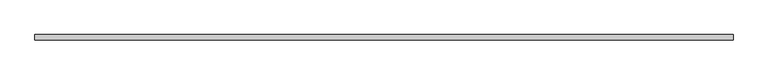
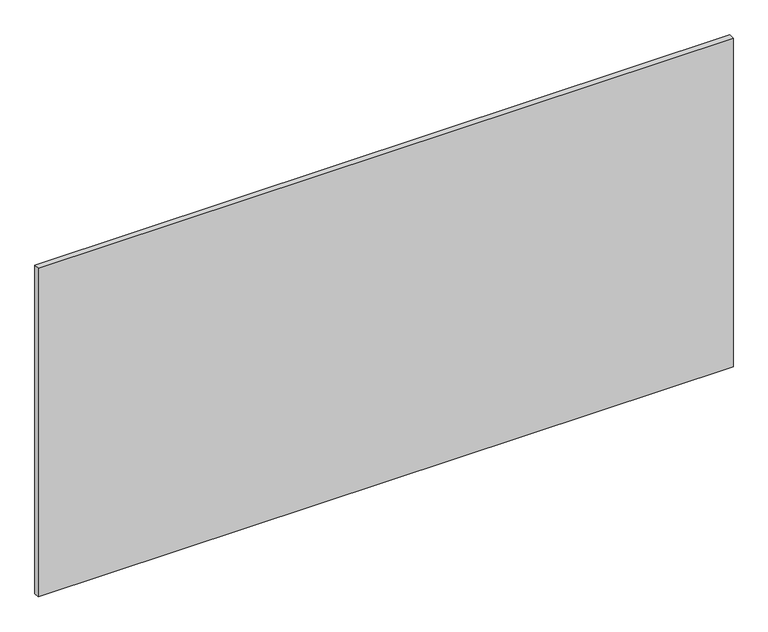
"""IFC4 building model written with IfcOpenShell, lengths in millimetres: proxy geometry, Inner panel:Inner panel:1:Inner panel:1 : Inner panel:Inner panel:300324:300043:Inner panel:1:Inner panel:1 : Inner panel:Inner panel:300324:300043 : Inner panel:Inner panel:1:Inner panel:1 : Inner panel:Inner panel:300324:300043:20 : Inner panel:Inner panel:1:Inner panel:1 : Inner panel:Inner panel:300324:300043:Inner panel:1:Inner panel:1 : Inner panel:Inner panel:300324:300043 : Inner panel:Inner panel:1:Inner panel:1 : Inner panel:Inner panel:300324:300043:300031."""

from ifc_helpers import new_model, si_unit, frame, origin, place, context, project, spatial, polyline, outline, extrude, source, transform, mapped, element, save


def generic_models_23cc8b8a(model_context):
    return source(origin(), model_context, "Body", "SweptSolid", [
        extrude(outline(polyline([(592512.5367239, -568186.6413841), (594950.9367239, -568186.6413841), (594950.9367239, -568205.6913841), (592512.5367239, -568205.6913841), (592512.5367239, -568186.6413841)])), frame((0.0, 0.0, 3721.1), z_axis=(0.0, 0.0, 1.0), x_axis=(1.0, 0.0, 0.0)), (0.0, 0.0, 1.0), 1219.2),
    ])


if __name__ == "__main__":
    model = new_model("IFC4")
    model_context = context("Model", 3, world=origin())
    ifc_project = project(units=[si_unit("LENGTHUNIT", "METRE", prefix="MILLI")], contexts=[model_context])
    site = spatial("IfcSite", under=ifc_project)
    building = spatial("IfcBuilding", under=site)
    placement = place(None, origin())
    generic_models_shape = generic_models_23cc8b8a(model_context)
    element("IfcBuildingElementProxy", 1, Name="Inner panel:Inner panel:1:Inner panel:1 : Inner panel:Inner panel:300324:300043:Inner panel:1:Inner panel:1 : Inner panel:Inner panel:300324:300043 : Inner panel:Inner panel:1:Inner panel:1 : Inner panel:Inner panel:300324:300043:20 : Inner panel:Inner panel:1:Inner panel:1 : Inner panel:Inner panel:300324:300043:Inner panel:1:Inner panel:1 : Inner panel:Inner panel:300324:300043 : Inner panel:Inner panel:1:Inner panel:1 : Inner panel:Inner panel:300324:300043:300031", ObjectType="Inner panel:Inner panel:1:Inner panel:1 : Inner panel:Inner panel:300324:300043:Inner panel:1:Inner panel:1 : Inner panel:Inner panel:300324:300043 : Inner panel:Inner panel:1:Inner panel:1 : Inner panel:Inner panel:300324:300043:20 : Inner panel:Inner panel:1:Inner panel:1 : Inner panel:Inner panel:300324:300043:Inner panel:1:Inner panel:1 : Inner panel:Inner panel:300324:300043 : Inner panel:Inner panel:1:Inner panel:1 : Inner panel:Inner panel:300324:300043:300031", at=placement, inside=building, context=model_context, shape_type="MappedRepresentation", body=[
        mapped(generic_models_shape, transform((0.0, 0.0, 0.0), x_axis=(1.0, 0.0, 0.0), y_axis=(0.0, 1.0, 0.0), z_axis=(0.0, 0.0, 1.0))),
    ])
    save(model, "model.ifc")

# Revit data of these elements
# Type "Inner panel:Inner panel:1:Inner panel:1 : Inner panel:Inner panel:300324:300043:Inner panel:1:Inner panel:1 : Inner panel:Inner panel:300324:300043 : Inner panel:Inner panel:1:Inner panel:1 : Inner panel:Inner panel:300324:300043:20 : Inner panel:Inner panel:1:Inner panel:1 : Inner panel:Inner panel:300324:300043:Inner panel:1:Inner panel:1 : Inner panel:Inner panel:300324:300043 : Inner panel:Inner panel:1:Inner panel:1 : Inner panel:Inner panel:300324:300043:300031"
#   NameOverride = "Inner panel:Inner panel:1:Inner panel:1 : Inner panel:Inner panel:300324:300043:Inner panel:1:Inner panel:1 : Inner panel:Inner panel:300324:300043 : Inner panel:Inner panel:1:Inner panel:1 : Inner panel:Inner panel:300324:300043:300031"
#   ObjectTypeOverride = "Inner panel:1:Inner panel:1 : Inner panel:Inner panel:300324:300043 : Inner panel:Inner panel:1:Inner panel:1 : Inner panel:Inner panel:300324:300043"
#   Reference = "Inner panel"
#   Tag = "300031"
# Element 1 (IfcBuildingElementProxy, "Inner panel:Inner panel:1:Inner panel:1 : Inner panel:Inner panel:300324:300043:Inner panel:1:Inner panel:1 : Inner panel:Inner panel:300324:300043 : Inner panel:Inner panel:1:Inner panel:1 : Inner panel:Inner panel:300324:300043:20 : Inner panel:Inner panel:1:Inner panel:1 : Inner panel:Inner panel:300324:300043:Inner panel:1:Inner panel:1 : Inner panel:Inner panel:300324:300043 : Inner panel:Inner panel:1:Inner panel:1 : Inner panel:Inner panel:300324:300043:300031")
#   Materials on its faces: "3/4\" PREFINISHED STAINED/SEALED PLYWOOD (FINISH: GRADE B,  FLAME SPREAD: CLASS B)"
# Materials
#   "3/4\" PREFINISHED STAINED/SEALED PLYWOOD (FINISH: GRADE B,  FLAME SPREAD: CLASS B)": class "Wood", colour RGB 149 120 74, transparency 0, Description = "Plywood, sheathing grade", Cost = 0
